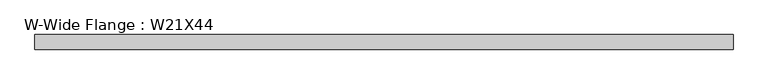
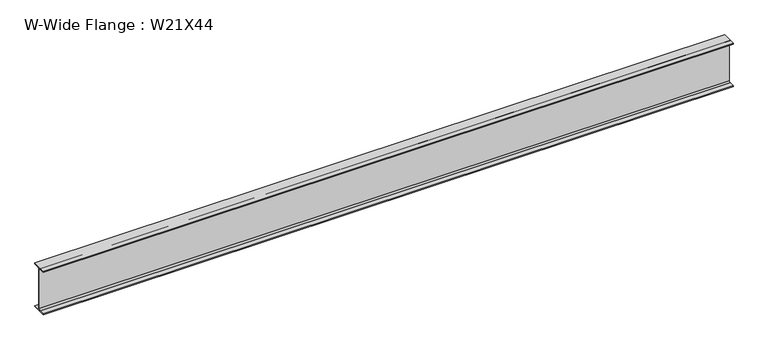
"""IFC4 building model written with IfcOpenShell, lengths in millimetres: beam geometry, W-Wide Flange : W21X44."""

from ifc_helpers import new_model, si_unit, point, frame, frame_2d, origin, place, context, project, spatial, polyline, circle_curve, trimmed, segment, composite_curve, outline, extrude, source, transform, mapped, element, save


def w_wide_flange_w21x44_7aeec852(model_context):
    return source(origin(), model_context, "Body", "SweptSolid", [
        extrude(outline(composite_curve([segment(polyline([(82.55, -251.46), (82.55, -262.89), (-82.55, -262.89), (-82.55, -251.46), (-21.59, -251.46)]), True, "CONTINUOUS"), segment(trimmed(circle_curve(frame_2d((-21.59, -234.315)), 17.145), [point((-21.59, -251.46))], [point((-4.445, -234.315))], True, "CARTESIAN"), True, "CONTINUOUS"), segment(polyline([(-4.445, -234.315), (-4.445, 234.315)]), True, "CONTINUOUS"), segment(trimmed(circle_curve(frame_2d((-21.59, 234.315)), 17.145), [point((-4.445, 234.315))], [point((-21.59, 251.46))], True, "CARTESIAN"), True, "CONTINUOUS"), segment(polyline([(-21.59, 251.46), (-82.55, 251.46), (-82.55, 262.89), (82.55, 262.89), (82.55, 251.46), (21.59, 251.46)]), True, "CONTINUOUS"), segment(trimmed(circle_curve(frame_2d((21.59, 234.315)), 17.145), [point((21.59, 251.46))], [point((4.445, 234.315))], True, "CARTESIAN"), True, "CONTINUOUS"), segment(polyline([(4.445, 234.315), (4.445, -234.315)]), True, "CONTINUOUS"), segment(trimmed(circle_curve(frame_2d((21.59, -234.315)), 17.145), [point((4.445, -234.315))], [point((21.59, -251.46))], True, "CARTESIAN"), True, "CONTINUOUS"), segment(polyline([(21.59, -251.46), (82.55, -251.46)]), True, "CONTINUOUS")], self_intersect=False)), frame((-3902.7822091, 0.0, 0.0), z_axis=(1.0, 0.0, 0.0), x_axis=(0.0, 1.0, 0.0)), (0.0, 0.0, 1.0), 7866.2677304),
    ])


if __name__ == "__main__":
    model = new_model("IFC4")
    model_context = context("Model", 3, world=origin())
    ifc_project = project(units=[si_unit("LENGTHUNIT", "METRE", prefix="MILLI")], contexts=[model_context])
    site = spatial("IfcSite", under=ifc_project)
    building = spatial("IfcBuilding", under=site)
    placement = place(None, origin())
    w_wide_flange_w21x44_shape = w_wide_flange_w21x44_7aeec852(model_context)
    element("IfcBeam", 1, ObjectType="W-Wide Flange : W21X44", at=placement, inside=building, context=model_context, shape_type="MappedRepresentation", body=[
        mapped(w_wide_flange_w21x44_shape, transform((0.0, 0.0, 0.0), x_axis=(1.0, 0.0, 0.0), y_axis=(0.0, 1.0, 0.0), z_axis=(0.0, 0.0, 1.0))),
    ])
    save(model, "model.ifc")

# Revit data of these elements
# Type "W-Wide Flange : W21X44"
#   Assembly Code = "B10"
#   W = 44
#   Length [instance default] = 1524 mm
#   bf = 165.1 mm
#   d = 525.78 mm
#   k = 28.575 mm
#   k2 = 17.145 mm
#   tf = 11.43 mm
#   tw = 8.89 mm
#   A = 0.00838708 m²
#   Structural Material [instance default] = Steel ASTM A992
# Element 1 (IfcBeam, "W-Wide Flange : W21X44")
#   Structural Material = Aluminum, Anodized Red
#   Materials on its faces: "Aluminum, Anodized Red"
# Materials
#   "Steel ASTM A992": class "Metal", colour RGB 128 0 0, transparency 0, Description = "Structural steel 50ksi", Cost = 0
#   "Aluminum, Anodized Red": class "Metal", colour RGB 120 120 120, transparency 0, Description = "Anodized aluminum, red", Cost = 0
